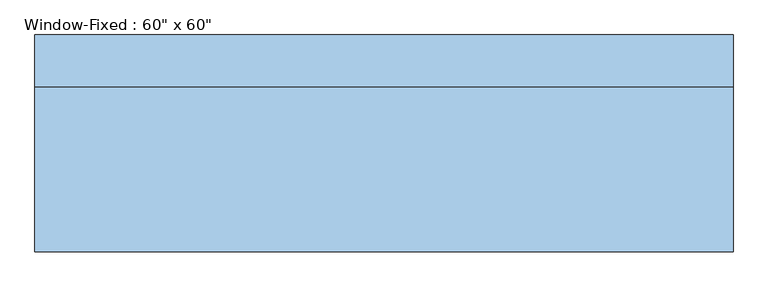
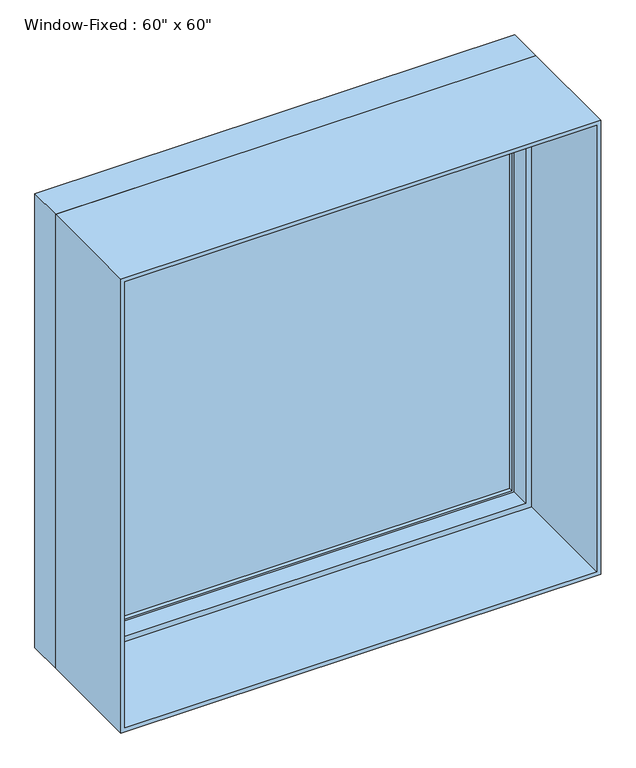
"""IFC4 building model written with IfcOpenShell, lengths in millimetres: window geometry."""

from ifc_helpers import new_model, si_unit, frame, origin, place, context, project, spatial, polyline, outline, extrude, faceted_brep, source, transform, mapped, element, save


def window_45f0c9e0(model_context):
    return source(origin(), model_context, "Body", "SolidModel", [
        extrude(outline(polyline([(723.9, 227.0125), (723.9, 220.6625), (-723.9, 220.6625), (-723.9, 227.0125), (723.9, 227.0125)])), frame((0.0, 0.0, 952.5), z_axis=(0.0, 0.0, 1.0), x_axis=(1.0, 0.0, 0.0)), (0.0, 0.0, 1.0), 1447.8),
        extrude(outline(polyline([(-723.9, 207.9625), (-723.9, 214.3125), (723.9, 214.3125), (723.9, 207.9625), (-723.9, 207.9625)])), frame((0.0, 0.0, 952.5), z_axis=(0.0, 0.0, 1.0), x_axis=(1.0, 0.0, 0.0)), (0.0, 0.0, 1.0), 1447.8),
        extrude(outline(polyline([(927.1, 749.3), (2425.7, 749.3), (2425.7, -749.3), (927.1, -749.3), (927.1, 749.3)]), holes=[polyline([(952.5, -723.9), (2400.3, -723.9), (2400.3, 723.9), (952.5, 723.9), (952.5, -723.9)])]), frame((0.0, 195.2625, 0.0), z_axis=(0.0, 1.0, 0.0), x_axis=(0.0, 0.0, 1.0)), (0.0, 0.0, 1.0), 44.45),
        extrude(outline(polyline([(2438.4, -762.0), (914.4, -762.0), (914.4, 762.0), (2438.4, 762.0), (2438.4, -762.0)]), holes=[polyline([(2425.7, 749.3), (927.1, 749.3), (927.1, -749.3), (2425.7, -749.3), (2425.7, 749.3)])]), frame((0.0, -227.0125, 0.0), z_axis=(0.0, 1.0, 0.0), x_axis=(0.0, 0.0, 1.0)), (0.0, 0.0, 1.0), 358.775),
        faceted_brep([(762.0, 131.7625, 2438.4), (762.0, 246.0625, 2438.4), (-762.0, 246.0625, 2438.4), (-762.0, 131.7625, 2438.4), (-762.0, 246.0625, 914.4), (-762.0, 131.7625, 914.4), (762.0, 246.0625, 914.4), (762.0, 131.7625, 914.4), (730.25, 131.7625, 2406.65), (730.25, 131.7625, 946.15), (-730.25, 131.7625, 946.15), (-730.25, 131.7625, 2406.65), (-749.3, 246.0625, 2425.7), (-749.3, 246.0625, 927.1), (749.3, 246.0625, 927.1), (749.3, 246.0625, 2425.7), (730.25, 195.2625, 2406.65), (-730.25, 195.2625, 2406.65), (749.3, 195.2625, 2425.7), (-749.3, 195.2625, 2425.7), (-730.25, 195.2625, 946.15), (-749.3, 195.2625, 927.1), (730.25, 195.2625, 946.15), (749.3, 195.2625, 927.1)], [[[0, 1, 2, 3]], [[3, 2, 4, 5]], [[5, 4, 6, 7]], [[3, 5, 7, 0], [8, 9, 10, 11]], [[7, 6, 1, 0]], [[1, 6, 4, 2], [12, 13, 14, 15]], [[16, 8, 11, 17]], [[15, 18, 19, 12]], [[17, 11, 10, 20]], [[12, 19, 21, 13]], [[20, 10, 9, 22]], [[13, 21, 23, 14]], [[22, 9, 8, 16]], [[18, 23, 21, 19], [17, 20, 22, 16]], [[14, 23, 18, 15]]]),
    ])


if __name__ == "__main__":
    model = new_model("IFC4")
    model_context = context("Model", 3, world=origin())
    ifc_project = project(units=[si_unit("LENGTHUNIT", "METRE", prefix="MILLI")], contexts=[model_context])
    site = spatial("IfcSite", under=ifc_project)
    building = spatial("IfcBuilding", under=site)
    placement = place(None, origin())
    window_shape = window_45f0c9e0(model_context)
    element("IfcWindow", 1, ObjectType="Window-Fixed : 60\" x 60\"", at=placement, inside=building, context=model_context, shape_type="MappedRepresentation", body=[
        mapped(window_shape, transform((0.0, 0.0, 0.0), x_axis=(1.0, 0.0, 0.0), y_axis=(0.0, 1.0, 0.0), z_axis=(0.0, 0.0, 1.0))),
    ])
    save(model, "model.ifc")

# Revit data of these elements
# Type "Window-Fixed : 60\" x 60\""
#   Type Mark = "WT-37"
#   Fire Rating = "0.5h"
#   Assembly Code = "B2020100"
#   Analytic Construction = "Double glazing - domestic"
#   Window Inset [instance default] = 0' - 0"
#   Wall Thickness [instance default] = 0' - 6"
#   Visual Light Transmittance = 0.81
#   Thermal Resistance (R) = 1.8146 (h·ft²·°F)/BTU
#   Solar Heat Gain Coefficient = 0.76
#   Rough Width = 5' - 0 1/2"
#   Rough Height = 5' - 0 1/2"
#   Interior Wall Closure [instance default] = 0' - 2 1/4"
#   Height = 5' - 0"
#   Heat Transfer Coefficient (U) = 0.5511 BTU/(h·ft²·°F)
#   Frame Extension [instance default] = 0' - 0 1/4"
#   Exterior Wall Closure [instance default] = 0' - 1 1/4"
#   Extension Jamb [instance default] = 0' - 2 1/4"
#   Default Sill Height = 3' - 0"
#   Width = 5' - 0"
#   Muntin Visibility = no
#   Interior Trim Visibility [instance default] = yes
#   Exterior Trim Visibility [instance default] = yes
#   Extension Jamb Visibility [instance default] = yes
#   Muntin Pattern = Muntin Pattern_2x2 : Muntin Pattern_2x2
#   Interior Trim Material = Wood - Stained
#   Interior Trim = Trim-Window-Interior-Flat : Picture Frame
#   Interior Frame Material = Wood - Stained
#   Glass Panel Material = Glass
#   Exterior Trim Material = Clad - White
#   Exterior Trim = Trim-Window-Exterior-Flat : with Sill
#   Exterior Frame Material = Clad - White
#   Wall Closure = (empty or 0)
# Element 1 (IfcWindow, "Window-Fixed : 60\" x 60\"")
#   Wall Thickness = 1' - 5 7/8"
#   Extension Jamb = 1' - 2 1/8"
#   Materials on its faces: "Wood - Stained", "Glass", "Clad - White"
# Materials
#   "Wood - Stained": class "Wood", colour RGB 224 178 126, transparency 0, Cost = 0
#   "Glass": class "Glass", colour RGB 0 128 192, transparency 0.75, Description = "Soda Lime Glass", Cost = 0
#   "Clad - White": class "Wood", colour RGB 242 242 238, transparency 0, Cost = 0
